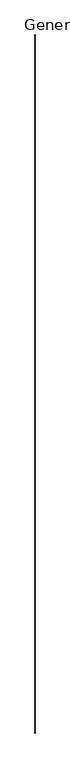
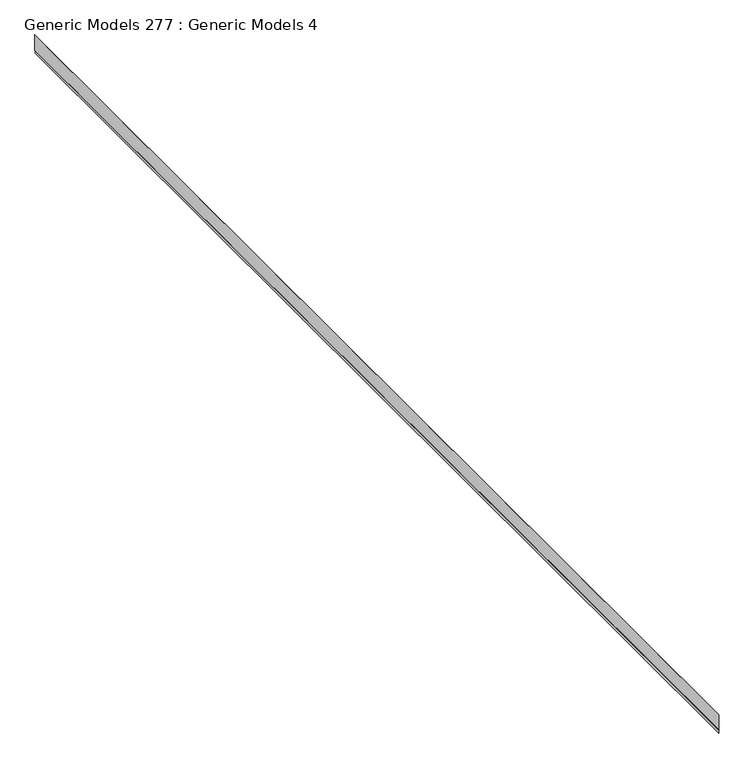
"""IFC4 building model written with IfcOpenShell, lengths in millimetres: proxy geometry, Generic Models 277 : Generic Models 4."""

import ifcopenshell
import ifcopenshell.guid

model = None  # the IFC model being written
_history = None  # IfcOwnerHistory: only IFC2X3 demands one
_inside = {}  # id of a spatial element -> (the spatial element, [elements in it])
_under = {}  # id of a project, library or spatial element -> (it, [spatial elements below it])
_declared = {}  # id of a project -> (the project, [libraries it declares])
_typed = {}  # id of a type object -> (the type object, [elements of that type])
_made_of = {}  # id of a material, layer set ... -> (it, [elements and type objects made of it])


def new_model(schema):
    """Start an empty IFC model of exactly this schema.

    Asked for "IFC4X3", IfcOpenShell would pick the latest addendum, in which some entities
    have other attributes; the version numbers below select the first issue.
    IFC2X3 requires an IfcOwnerHistory on every rooted entity: one is made here for all.
    """
    global model, _history
    if schema == "IFC4X3":
        model = ifcopenshell.file(schema_version=(4, 3, 0, 0))
    else:
        model = ifcopenshell.file(schema=schema)
    _inside.clear()
    _under.clear()
    _declared.clear()
    _typed.clear()
    _made_of.clear()
    _history = None
    if model.schema == "IFC2X3":
        org = make("IfcOrganization", Name="unknown")
        user = make(
            "IfcPersonAndOrganization",
            ThePerson=make("IfcPerson", FamilyName="unknown"),
            TheOrganization=org,
        )
        app = make(
            "IfcApplication",
            ApplicationDeveloper=org,
            Version="unknown",
            ApplicationFullName="unknown",
            ApplicationIdentifier="unknown",
        )
        _history = make(
            "IfcOwnerHistory",
            OwningUser=user,
            OwningApplication=app,
            ChangeAction="ADDED",
            CreationDate=0,
        )
    return model


def make(cls, **values):
    """One entity of the class cls with the attributes given. An attribute that is None is left unset."""
    return model.create_entity(
        cls, **{name: value for name, value in values.items() if value is not None}
    )


def rooted(cls, **values):
    """An entity with a GlobalId (a new one), such as an element, a storey or a relation."""
    return make(cls, GlobalId=ifcopenshell.guid.new(), OwnerHistory=_history, **values)


def si_unit(unit_type, name, prefix=None):
    """IfcSIUnit, for example si_unit("LENGTHUNIT", "METRE", prefix="MILLI")."""
    return make("IfcSIUnit", UnitType=unit_type, Prefix=prefix, Name=name)


def assignment(units):
    """IfcUnitAssignment: the units of a project."""
    return None if units is None else make("IfcUnitAssignment", Units=units)


def point(xyz):
    """IfcCartesianPoint."""
    return None if xyz is None else make("IfcCartesianPoint", Coordinates=xyz)


def direction(xyz):
    """IfcDirection."""
    return None if xyz is None else make("IfcDirection", DirectionRatios=xyz)


def frame(location, z_axis=None, x_axis=None):
    """IfcAxis2Placement3D, a coordinate frame: its origin and axes. An axis left out is left unset."""
    return make(
        "IfcAxis2Placement3D",
        Location=point(location),
        Axis=direction(z_axis),
        RefDirection=direction(x_axis),
    )


def origin():
    """The frame at (0, 0, 0) with its axes left unset."""
    return frame((0.0, 0.0, 0.0))


def place(relative_to, where):
    """IfcLocalPlacement: puts the frame where relative to a parent placement (None: the world)."""
    return make(
        "IfcLocalPlacement", PlacementRelTo=relative_to, RelativePlacement=where
    )


def context(
    kind, dimensions, precision=None, world=None, true_north=None, identifier=None
):
    """IfcGeometricRepresentationContext, for example the 3D "Model" context."""
    return make(
        "IfcGeometricRepresentationContext",
        ContextIdentifier=identifier,
        ContextType=kind,
        CoordinateSpaceDimension=dimensions,
        Precision=precision,
        WorldCoordinateSystem=world,
        TrueNorth=true_north,
    )


def project(units=None, contexts=None):
    """IfcProject with its units and contexts."""
    return rooted(
        "IfcProject",
        Name="project",
        RepresentationContexts=contexts,
        UnitsInContext=assignment(units),
    )


def spatial(cls, under=None, at=None, **own):
    """A site, building, storey or space (cls), placed at a placement, below another one or the project."""
    s = rooted(cls, ObjectPlacement=at, **own)
    if under is not None:
        _under.setdefault(under.id(), (under, []))[1].append(s)
    return s


def polyline(points):
    """IfcPolyline through the points."""
    return make("IfcPolyline", Points=[point(p) for p in points])


def outline(outer, holes=None, kind="AREA"):
    """IfcArbitraryClosedProfileDef: a profile drawn as a closed curve; with holes, ...WithVoids."""
    if holes is None:
        return make("IfcArbitraryClosedProfileDef", ProfileType=kind, OuterCurve=outer)
    return make(
        "IfcArbitraryProfileDefWithVoids",
        ProfileType=kind,
        OuterCurve=outer,
        InnerCurves=holes,
    )


def extrude(swept, where, along, depth):
    """IfcExtrudedAreaSolid: the profile swept, set in the frame where, extruded along a direction by depth."""
    return make(
        "IfcExtrudedAreaSolid",
        SweptArea=swept,
        Position=where,
        ExtrudedDirection=direction(along),
        Depth=depth,
    )


def shape(context_of_items, identifier, shape_type, items):
    """IfcShapeRepresentation: the items that make up one representation, for example the "Body"."""
    return make(
        "IfcShapeRepresentation",
        ContextOfItems=context_of_items,
        RepresentationIdentifier=identifier,
        RepresentationType=shape_type,
        Items=items,
    )


def source(mapping_origin, context_of_items, identifier, shape_type, items):
    """IfcRepresentationMap: a shape defined once, which mapped items show again and again."""
    return make(
        "IfcRepresentationMap",
        MappingOrigin=mapping_origin,
        MappedRepresentation=shape(context_of_items, identifier, shape_type, items),
    )


def transform(
    local_origin,
    x_axis=None,
    y_axis=None,
    z_axis=None,
    scale=None,
    scale2=None,
    scale3=None,
    uniform=True,
):
    """IfcCartesianTransformationOperator3D, or its non-uniform kind. x_axis, y_axis, z_axis: its Axis1, 2, 3."""
    if uniform:
        return make(
            "IfcCartesianTransformationOperator3D",
            Axis1=direction(x_axis),
            Axis2=direction(y_axis),
            LocalOrigin=point(local_origin),
            Scale=scale,
            Axis3=direction(z_axis),
        )
    return make(
        "IfcCartesianTransformationOperator3DnonUniform",
        Axis1=direction(x_axis),
        Axis2=direction(y_axis),
        LocalOrigin=point(local_origin),
        Scale=scale,
        Axis3=direction(z_axis),
        Scale2=scale2,
        Scale3=scale3,
    )


def mapped(mapping_source, mapping_target):
    """IfcMappedItem: shows the shape of a source again, moved by a transform."""
    return make(
        "IfcMappedItem", MappingSource=mapping_source, MappingTarget=mapping_target
    )


def made_of(thing, what):
    """Note that an element or type object is made of a material, layer set ...; save() writes the relation."""
    if what is not None:
        _made_of.setdefault(what.id(), (what, []))[1].append(thing)
    return thing


def element(
    cls,
    number,
    at=None,
    inside=None,
    cuts=None,
    type_object=None,
    material=None,
    context=None,
    identifier="Body",
    shape_type=None,
    held_by="IfcProductDefinitionShape",
    body=None,
    shapes=None,
    **own,
):
    """One element of the class cls, such as IfcWall. Its Tag is "e" and its number.

    at: its placement. inside: the storey or other place that contains it. cuts: it is an
    opening in that element (IfcRelVoidsElement). A single representation is given by context,
    identifier, shape_type and body (its items); several are given by shapes. held_by: the class
    of the entity that holds the representations. save() writes the other relations.
    """
    e = rooted(cls, Tag="e%d" % number, ObjectPlacement=at, **own)
    if body is not None:
        shapes = [shape(context, identifier, shape_type, body)]
    if shapes is not None:
        e.Representation = make(held_by, Representations=shapes)
    if inside is not None:
        _inside.setdefault(inside.id(), (inside, []))[1].append(e)
    if cuts is not None:
        rooted(
            "IfcRelVoidsElement", RelatingBuildingElement=cuts, RelatedOpeningElement=e
        )
    if type_object is not None:
        _typed.setdefault(type_object.id(), (type_object, []))[1].append(e)
    return made_of(e, material)


def aggregate(whole, parts):
    """IfcRelAggregates: a whole, such as a stair, and the parts it consists of."""
    return rooted("IfcRelAggregates", RelatingObject=whole, RelatedObjects=parts)


def save(model, path):
    """Write the relations noted so far, then the file.

    IfcRelAggregates (storeys below a building ...), IfcRelContainedInSpatialStructure (elements
    in a storey), IfcRelDefinesByType, IfcRelAssociatesMaterial and IfcRelDeclares: one each for
    every whole, place, type object, material and project.
    """
    for whole, parts in _under.values():
        aggregate(whole, parts)
    for where, things in _inside.values():
        rooted(
            "IfcRelContainedInSpatialStructure",
            RelatedElements=things,
            RelatingStructure=where,
        )
    for kind, things in _typed.values():
        rooted("IfcRelDefinesByType", RelatedObjects=things, RelatingType=kind)
    for what, things in _made_of.values():
        rooted("IfcRelAssociatesMaterial", RelatedObjects=things, RelatingMaterial=what)
    for by, libraries in _declared.values():
        rooted("IfcRelDeclares", RelatingContext=by, RelatedDefinitions=libraries)
    model.write(path)


def generic_models_277_generic_models_4_b8a13d6f(model_context):
    return source(origin(), model_context, "Body", "SweptSolid", [
        extrude(outline(polyline([(126311.4404211, 1638.8605335), (126305.7987003, 1640.9139519), (126258.231851, 1640.9139519), (126258.231851, 1641.7077019), (126305.9386599, 1641.7077019), (126311.5803806, 1639.6542835), (126564.9652101, 1639.6542835), (126564.9652101, 1638.8605335), (126311.4404211, 1638.8605335)])), frame((0.0, -9028.6126687, 0.0), z_axis=(0.0, 1.0, 0.0), x_axis=(0.0, 0.0, 1.0)), (0.0, 0.0, 1.0), 18643.6),
    ])


if __name__ == "__main__":
    model = new_model("IFC4")
    model_context = context("Model", 3, world=origin())
    ifc_project = project(units=[si_unit("LENGTHUNIT", "METRE", prefix="MILLI")], contexts=[model_context])
    site = spatial("IfcSite", under=ifc_project)
    building = spatial("IfcBuilding", under=site)
    placement = place(None, origin())
    generic_models_277_generic_models_4_shape = generic_models_277_generic_models_4_b8a13d6f(model_context)
    element("IfcBuildingElementProxy", 1, Name="Generic Models 277 : Generic Models 4", ObjectType="Generic Models 277 : Generic Models 4", at=placement, inside=building, context=model_context, shape_type="MappedRepresentation", body=[
        mapped(generic_models_277_generic_models_4_shape, transform((0.0, 0.0, 0.0), x_axis=(1.0, 0.0, 0.0), y_axis=(0.0, 1.0, 0.0), z_axis=(0.0, 0.0, 1.0))),
    ])
    save(model, "model.ifc")

# Revit data of these elements
# Element 1 (IfcBuildingElementProxy, "Generic Models 277 : Generic Models 4")
#   Materials on its faces: "_DRAINABLE BUILDING WRAP"
# Materials
#   "_DRAINABLE BUILDING WRAP": class "Generic", colour RGB 67 154 161, transparency 0, Cost = 0
